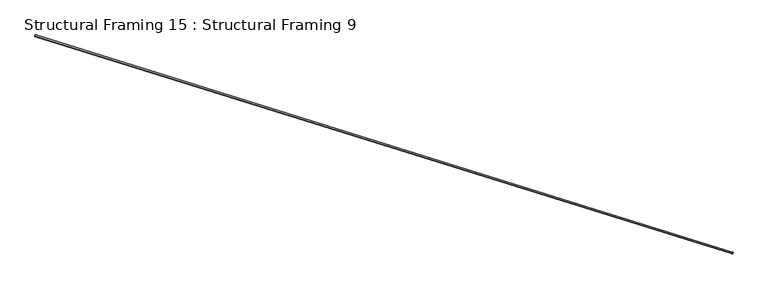
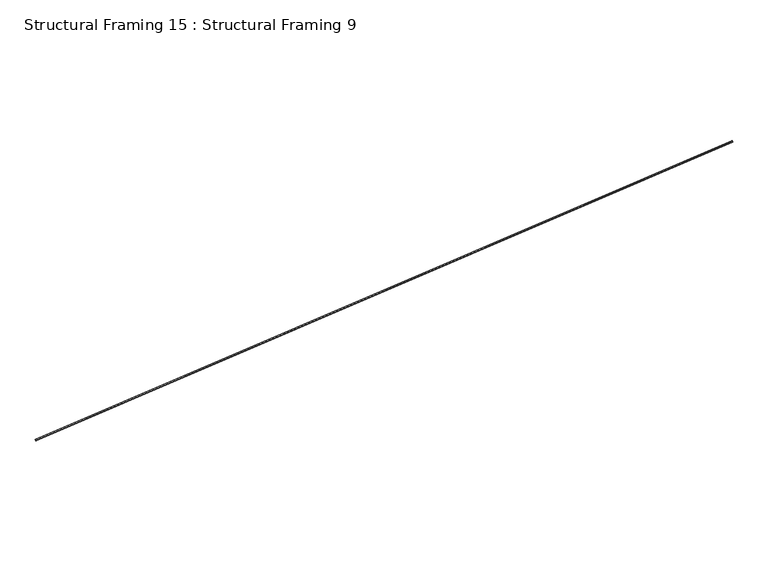
"""IFC4 building model written with IfcOpenShell, lengths in millimetres: beam geometry, Structural Framing 15 : Structural Framing 9."""

from ifc_helpers import new_model, si_unit, point, frame, origin, origin_2d, place, context, project, spatial, circle_curve, trimmed, segment, composite_curve, outline, extrude, source, transform, mapped, element, save


def structural_framing_15_structural_framing_9_7626a4d9(model_context):
    return source(origin(), model_context, "Body", "SweptSolid", [
        extrude(outline(composite_curve([segment(trimmed(circle_curve(origin_2d(), 6.35), [point((0.0, 6.35))], [point((0.0, -6.35))], False, "CARTESIAN"), True, "CONTINUOUS"), segment(trimmed(circle_curve(origin_2d(), 6.35), [point((0.0, -6.35))], [point((0.0, 6.35))], False, "CARTESIAN"), True, "CONTINUOUS")], self_intersect=False)), frame((12608.4580052, 11688.3780277, 2959.3363832), z_axis=(0.8989286779363523, -0.28046158673269883, 0.3365539040792405), x_axis=(0.0, -0.7682212795973774, -0.6401843996644779)), (0.0, 0.0, 1.0), 5845.7129347),
    ])


if __name__ == "__main__":
    model = new_model("IFC4")
    model_context = context("Model", 3, world=origin())
    ifc_project = project(units=[si_unit("LENGTHUNIT", "METRE", prefix="MILLI")], contexts=[model_context])
    site = spatial("IfcSite", under=ifc_project)
    building = spatial("IfcBuilding", under=site)
    placement = place(None, origin())
    structural_framing_15_structural_framing_9_shape = structural_framing_15_structural_framing_9_7626a4d9(model_context)
    element("IfcBeam", 1, ObjectType="Structural Framing 15 : Structural Framing 9", at=placement, inside=building, context=model_context, shape_type="MappedRepresentation", body=[
        mapped(structural_framing_15_structural_framing_9_shape, transform((0.0, 0.0, 0.0), x_axis=(1.0, 0.0, 0.0), y_axis=(0.0, 1.0, 0.0), z_axis=(0.0, 0.0, 1.0))),
    ])
    save(model, "model.ifc")

# Revit data of these elements
# Type "Structural Framing 15 : Structural Framing 9"
#   Structural Material [instance default] = EXISTING LATERAL BRACING (1/4" CABLE)
# Element 1 (IfcBeam, "Structural Framing 15 : Structural Framing 9")
#   Materials on its faces: "EXISTING LATERAL BRACING (1/4\" CABLE)"
# Materials
#   "EXISTING LATERAL BRACING (1/4\" CABLE)": class "Generic", colour RGB 120 120 120, transparency 0, Cost = 0
